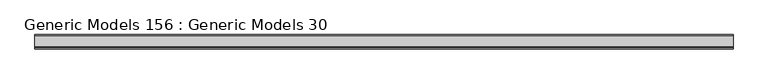
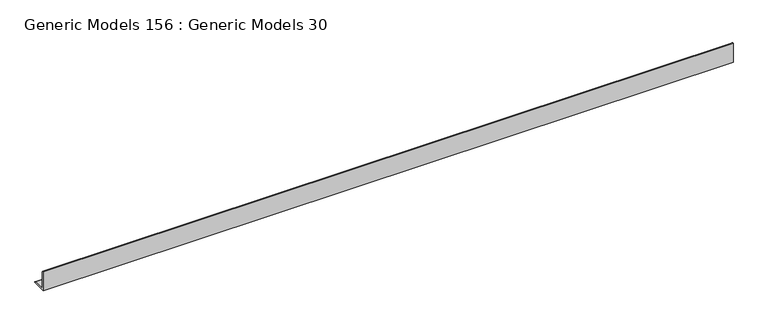
"""IFC4 building model written with IfcOpenShell, lengths in millimetres: proxy geometry, Generic Models 156 : Generic Models 30."""

from ifc_helpers import new_model, si_unit, point, frame, frame_2d, origin, place, context, project, spatial, polyline, circle_curve, trimmed, segment, composite_curve, outline, extrude, source, transform, mapped, element, save


def generic_models_156_generic_models_30_2a2f6dbc(model_context):
    return source(origin(), model_context, "Body", "SweptSolid", [
        extrude(outline(composite_curve([segment(polyline([(40981.6481612, 268859.0544757), (40981.6481612, 268947.9544757)]), True, "CONTINUOUS"), segment(trimmed(circle_curve(frame_2d((40981.6481612, 268941.6044757)), 6.35), [point((40981.6481612, 268947.9544757))], [point((40987.9981612, 268941.6044757))], False, "CARTESIAN"), True, "CONTINUOUS"), segment(polyline([(40987.9981612, 268941.6044757), (40987.9981612, 268871.7544757)]), True, "CONTINUOUS"), segment(trimmed(circle_curve(frame_2d((40994.3481612, 268871.7544757)), 6.35), [point((40987.9981612, 268871.7544757))], [point((40994.3481612, 268865.4044757))], True, "CARTESIAN"), True, "CONTINUOUS"), segment(polyline([(40994.3481612, 268865.4044757), (41038.7981612, 268865.4044757)]), True, "CONTINUOUS"), segment(trimmed(circle_curve(frame_2d((41038.7981612, 268859.0544757)), 6.35), [point((41038.7981612, 268865.4044757))], [point((41045.1481612, 268859.0544757))], False, "CARTESIAN"), True, "CONTINUOUS"), segment(polyline([(41045.1481612, 268859.0544757), (40981.6481612, 268859.0544757)]), True, "CONTINUOUS")], self_intersect=False)), frame((32314.35773, 0.0, 0.0), z_axis=(1.0, 0.0, 0.0), x_axis=(0.0, 1.0, 0.0)), (0.0, 0.0, 1.0), 3048.0),
    ])


if __name__ == "__main__":
    model = new_model("IFC4")
    model_context = context("Model", 3, world=origin())
    ifc_project = project(units=[si_unit("LENGTHUNIT", "METRE", prefix="MILLI")], contexts=[model_context])
    site = spatial("IfcSite", under=ifc_project)
    building = spatial("IfcBuilding", under=site)
    placement = place(None, origin())
    generic_models_156_generic_models_30_shape = generic_models_156_generic_models_30_2a2f6dbc(model_context)
    element("IfcBuildingElementProxy", 1, Name="Generic Models 156 : Generic Models 30", ObjectType="Generic Models 156 : Generic Models 30", at=placement, inside=building, context=model_context, shape_type="MappedRepresentation", body=[
        mapped(generic_models_156_generic_models_30_shape, transform((0.0, 0.0, 0.0), x_axis=(1.0, 0.0, 0.0), y_axis=(0.0, 1.0, 0.0), z_axis=(0.0, 0.0, 1.0))),
    ])
    save(model, "model.ifc")

# Revit data of these elements
# Element 1 (IfcBuildingElementProxy, "Generic Models 156 : Generic Models 30")
#   Materials on its faces: "10FT GALV 3 1/2\"X 2 1/2\" X 1/4\" STEEL ANGLE"
# Materials
#   "10FT GALV 3 1/2\"X 2 1/2\" X 1/4\" STEEL ANGLE": class "Metal", colour RGB 199 199 199, transparency 0, Description = "Structural steel, ASTM A36 Grade B, mill finish", Cost = 0
